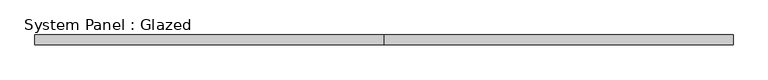
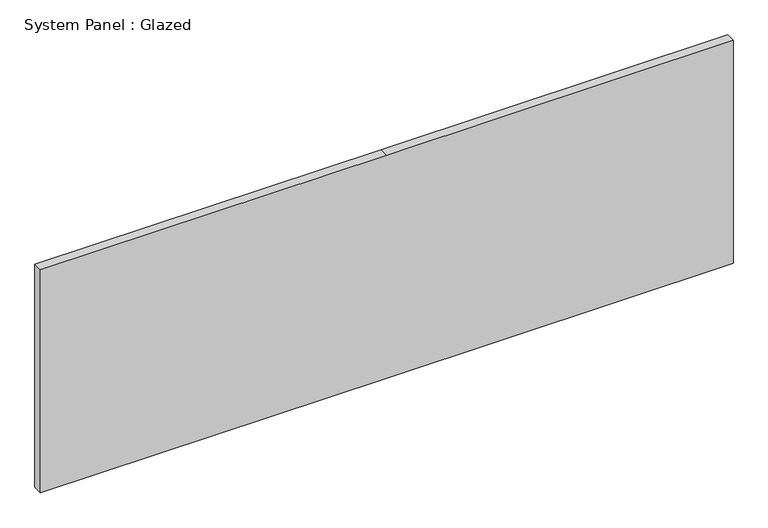
"""IFC4 building model written with IfcOpenShell, lengths in millimetres: plate geometry, System Panel : Glazed."""

from ifc_helpers import new_model, si_unit, frame, origin, place, context, project, spatial, polyline, outline, extrude, source, transform, mapped, element, save


def system_panel_glazed_8a60f612(model_context):
    return source(origin(), model_context, "Body", "SweptSolid", [
        extrude(outline(polyline([(0.0, -914.4), (0.0, 0.0), (0.0, 914.4), (622.3, 914.4), (622.3, 0.0), (622.3, -914.4), (0.0, -914.4)])), frame((0.0, 19.05, 0.0), z_axis=(0.0, 1.0, 0.0), x_axis=(0.0, 0.0, 1.0)), (0.0, 0.0, 1.0), 25.4),
    ])


if __name__ == "__main__":
    model = new_model("IFC4")
    model_context = context("Model", 3, world=origin())
    ifc_project = project(units=[si_unit("LENGTHUNIT", "METRE", prefix="MILLI")], contexts=[model_context])
    site = spatial("IfcSite", under=ifc_project)
    building = spatial("IfcBuilding", under=site)
    placement = place(None, origin())
    system_panel_glazed_shape = system_panel_glazed_8a60f612(model_context)
    element("IfcPlate", 1, ObjectType="System Panel : Glazed", at=placement, inside=building, context=model_context, shape_type="MappedRepresentation", body=[
        mapped(system_panel_glazed_shape, transform((0.0, 0.0, 0.0), x_axis=(1.0, 0.0, 0.0), y_axis=(0.0, 1.0, 0.0), z_axis=(0.0, 0.0, 1.0))),
    ])
    save(model, "model.ifc")

# Revit data of these elements
# Element 1 (IfcPlate, "System Panel : Glazed")
#   Materials on its faces: "Glass"
# Materials
#   "Glass": class "Glass", colour RGB 0 128 192, transparency 0.75
